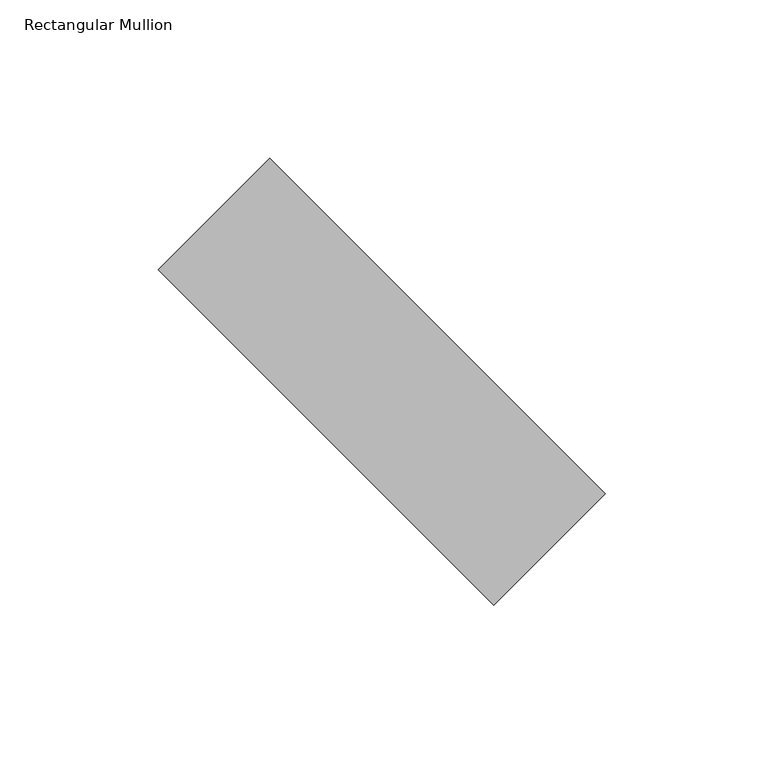
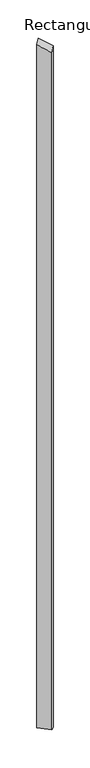
"""IFC4 building model written with IfcOpenShell, lengths in millimetres: member geometry, Rectangular Mullion : tilted mullions."""

from ifc_helpers import new_model, si_unit, origin, place, context, project, spatial, faceted_brep, source, transform, mapped, element, save


def rectangular_mullion_345c46c6(model_context):
    return source(origin(), model_context, "Body", "Brep", [
        faceted_brep([(-35.3553391, 70.7106781, -7999.7689278), (70.7106781, -35.3553391, -7999.7689278), (35.3553391, -70.7106781, -7999.7689278), (-70.7106781, 35.3553391, -7999.7689278), (-70.7106781, 35.3553391, 10.2368528), (-35.3553391, 70.7106781, 55.2243041), (35.3553391, -70.7106781, -55.2243041), (70.7106781, -35.3553391, -10.2368528)], [[[0, 1, 2, 3]], [[4, 5, 0, 3]], [[6, 4, 3, 2]], [[7, 6, 2, 1]], [[5, 7, 1, 0]], [[5, 4, 6, 7]]]),
    ])


if __name__ == "__main__":
    model = new_model("IFC4")
    model_context = context("Model", 3, world=origin())
    ifc_project = project(units=[si_unit("LENGTHUNIT", "METRE", prefix="MILLI")], contexts=[model_context])
    site = spatial("IfcSite", under=ifc_project)
    building = spatial("IfcBuilding", under=site)
    placement = place(None, origin())
    rectangular_mullion_shape = rectangular_mullion_345c46c6(model_context)
    element("IfcMember", 1, ObjectType="Rectangular Mullion : tilted mullions", at=placement, inside=building, context=model_context, shape_type="MappedRepresentation", body=[
        mapped(rectangular_mullion_shape, transform((0.0, 0.0, 0.0), x_axis=(1.0, 0.0, 0.0), y_axis=(0.0, 1.0, 0.0), z_axis=(0.0, 0.0, 1.0))),
    ])
    save(model, "model.ifc")

# Revit data of these elements
# Type "Rectangular Mullion : tilted mullions"
#   built-in parameter 1007304 = 0.492126 (stored number, unit not read)
#   built-in parameter 1007301 = 0.082021 (stored number, unit not read)
#   built-in parameter 1007300 = 0.082021 (stored number, unit not read)
# Element 1 (IfcMember, "Rectangular Mullion : tilted mullions")
#   Materials on its faces: "Aluminum"
# Materials
#   "Aluminum": class "Metal", colour RGB 244 244 244, transparency 0, Description = "Aluminum 6061", Cost = 0
